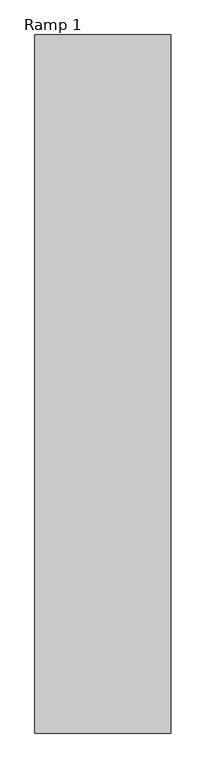
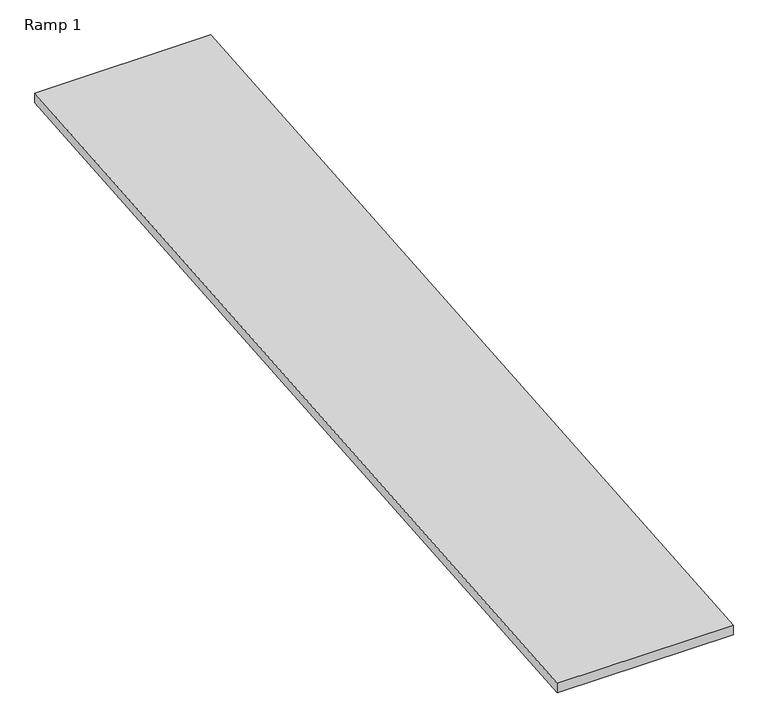
"""IFC4 building model written with IfcOpenShell, lengths in millimetres: ramp geometry, Ramp 1."""

from ifc_helpers import new_model, si_unit, frame, origin, place, context, project, spatial, polyline, outline, extrude, source, transform, mapped, element, save


def ramp_1_70fcbfb5(model_context):
    return source(origin(), model_context, "Body", "SweptSolid", [
        extrude(outline(polyline([(39498.9598199, -1200.0), (57498.9598198, 300.0), (57498.9598198, 99.306757), (39498.9598199, -1400.693243), (39498.9598199, -1200.0)])), frame((-7541.0, 0.0, 0.0), z_axis=(1.0, 0.0, 0.0), x_axis=(0.0, 1.0, 0.0)), (0.0, 0.0, 1.0), 3500.0),
    ])


if __name__ == "__main__":
    model = new_model("IFC4")
    model_context = context("Model", 3, world=origin())
    ifc_project = project(units=[si_unit("LENGTHUNIT", "METRE", prefix="MILLI")], contexts=[model_context])
    site = spatial("IfcSite", under=ifc_project)
    building = spatial("IfcBuilding", under=site)
    placement = place(None, origin())
    ramp_1_shape = ramp_1_70fcbfb5(model_context)
    element("IfcRamp", 1, ObjectType="Ramp 1", at=placement, inside=building, context=model_context, shape_type="MappedRepresentation", body=[
        mapped(ramp_1_shape, transform((0.0, 0.0, 0.0), x_axis=(1.0, 0.0, 0.0), y_axis=(0.0, 1.0, 0.0), z_axis=(0.0, 0.0, 1.0))),
    ])
    save(model, "model.ifc")
